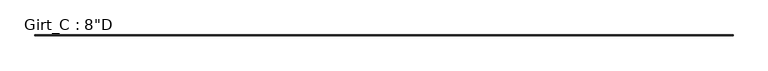
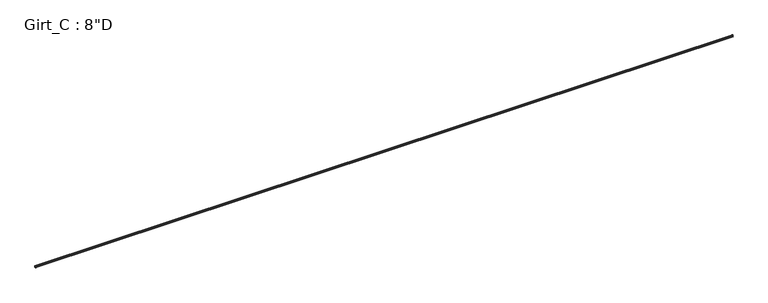
"""IFC4 building model written with IfcOpenShell, lengths in millimetres: beam geometry."""

from ifc_helpers import new_model, si_unit, point, frame, frame_2d, origin, place, context, project, spatial, polyline, circle_curve, trimmed, segment, composite_curve, outline, extrude, source, transform, mapped, element, save


def beam_8d9c0b98(model_context):
    return source(origin(), model_context, "Body", "SweptSolid", [
        extrude(outline(composite_curve([segment(polyline([(-87.5109375, 101.6), (-3.3734375, 101.6)]), True, "CONTINUOUS"), segment(trimmed(circle_curve(frame_2d((-3.3734375, 96.8375)), 4.7625), [point((-3.3734375, 101.6))], [point((1.3890625, 96.8375))], False, "CARTESIAN"), True, "CONTINUOUS"), segment(polyline([(1.3890625, 96.8375), (1.3890625, -96.8375)]), True, "CONTINUOUS"), segment(trimmed(circle_curve(frame_2d((-3.3734375, -96.8375)), 4.7625), [point((1.3890625, -96.8375))], [point((-3.3734375, -101.6))], False, "CARTESIAN"), True, "CONTINUOUS"), segment(polyline([(-3.3734375, -101.6), (-87.5109375, -101.6), (-99.7792647, -86.979177), (-97.6510975, -85.1934327), (-86.2154765, -98.821875), (-3.2694106, -98.821875)]), True, "CONTINUOUS"), segment(trimmed(circle_curve(frame_2d((-3.3748024, -96.8389339)), 1.9857399), [point((-3.2694106, -98.821875))], [point((-1.3890625, -96.8389339))], True, "CARTESIAN"), True, "CONTINUOUS"), segment(polyline([(-1.3890625, -96.8389339), (-1.3890625, 96.8381931)]), True, "CONTINUOUS"), segment(trimmed(circle_curve(frame_2d((-3.3741066, 96.8381931)), 1.9850441), [point((-1.3890625, 96.8381931))], [point((-3.3005807, 98.821875))], True, "CARTESIAN"), True, "CONTINUOUS"), segment(polyline([(-3.3005807, 98.821875), (-86.2154765, 98.821875), (-97.6278742, 85.221109), (-99.7560415, 87.0068534), (-87.5109375, 101.6)]), True, "CONTINUOUS")], self_intersect=False)), frame((-44450.0, 0.0, 0.0), z_axis=(1.0, 0.0, 0.0), x_axis=(0.0, 1.0, 0.0)), (0.0, 0.0, 1.0), 88900.0),
    ])


if __name__ == "__main__":
    model = new_model("IFC4")
    model_context = context("Model", 3, world=origin())
    ifc_project = project(units=[si_unit("LENGTHUNIT", "METRE", prefix="MILLI")], contexts=[model_context])
    site = spatial("IfcSite", under=ifc_project)
    building = spatial("IfcBuilding", under=site)
    placement = place(None, origin())
    beam_shape = beam_8d9c0b98(model_context)
    element("IfcBeam", 1, ObjectType="Girt_C : 8\"D", at=placement, inside=building, context=model_context, shape_type="MappedRepresentation", body=[
        mapped(beam_shape, transform((0.0, 0.0, 0.0), x_axis=(1.0, 0.0, 0.0), y_axis=(0.0, 1.0, 0.0), z_axis=(0.0, 0.0, 1.0))),
    ])
    save(model, "model.ifc")

# Revit data of these elements
# Type "Girt_C : 8\"D"
#   half leg = 0' - 1 3/4"
#   Web_Thickness = 0' - 0 7/64"
#   Length [instance default] = 10' - 0"
#   Leg_1 = 0' - 3 1/2"
#   Height = 0' - 8"
#   Structural Material [instance default] = none
# Element 1 (IfcBeam, "Girt_C : 8\"D")
#   Structural Material = CEE' SECTION (8.0x3.5C - SEE STRUCT. DWGS)
#   Materials on its faces: "CEE' SECTION (8.0x3.5C - SEE STRUCT. DWGS)"
# Materials
#   "CEE' SECTION (8.0x3.5C - SEE STRUCT. DWGS)": class "Metal", colour RGB 137 146 153, transparency 0, Description = "Steel, mill finish", Cost = 0
